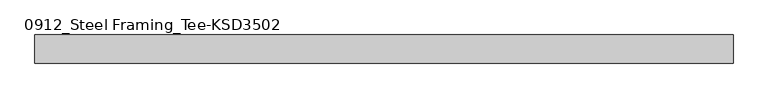
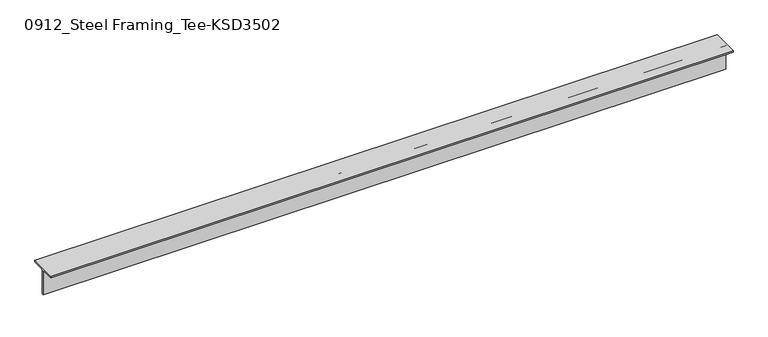
"""IFC4 building model written with IfcOpenShell, lengths in millimetres: member geometry, 0912_Steel Framing_Tee-KSD3502 : H_SB_ASB_CT-150x150x6.5x9."""

from ifc_helpers import new_model, si_unit, point, frame, frame_2d, origin, place, context, project, spatial, polyline, circle_curve, trimmed, segment, composite_curve, outline, extrude, source, transform, mapped, element, save


def member_0912_steel_framing_tee_ksd3502_bae0200a(model_context):
    return source(origin(), model_context, "Body", "SweptSolid", [
        extrude(outline(composite_curve([segment(polyline([(-75.0, 75.0), (75.0, 75.0), (75.0, 66.0), (16.25, 66.0)]), True, "CONTINUOUS"), segment(trimmed(circle_curve(frame_2d((16.25, 53.0)), 13.0), [point((16.25, 66.0))], [point((3.25, 53.0))], True, "CARTESIAN"), True, "CONTINUOUS"), segment(polyline([(3.25, 53.0), (3.25, -75.0), (-3.25, -75.0), (-3.25, 53.0)]), True, "CONTINUOUS"), segment(trimmed(circle_curve(frame_2d((-16.25, 53.0)), 13.0), [point((-3.25, 53.0))], [point((-16.25, 66.0))], True, "CARTESIAN"), True, "CONTINUOUS"), segment(polyline([(-16.25, 66.0), (-75.0, 66.0), (-75.0, 75.0)]), True, "CONTINUOUS")], self_intersect=False)), frame((-1887.85, 0.0, 0.0), z_axis=(1.0, 0.0, 0.0), x_axis=(0.0, 1.0, 0.0)), (0.0, 0.0, 1.0), 3728.1),
    ])


if __name__ == "__main__":
    model = new_model("IFC4")
    model_context = context("Model", 3, world=origin())
    ifc_project = project(units=[si_unit("LENGTHUNIT", "METRE", prefix="MILLI")], contexts=[model_context])
    site = spatial("IfcSite", under=ifc_project)
    building = spatial("IfcBuilding", under=site)
    placement = place(None, origin())
    member_0912_steel_framing_tee_ksd3502_shape = member_0912_steel_framing_tee_ksd3502_bae0200a(model_context)
    element("IfcMember", 1, ObjectType="0912_Steel Framing_Tee-KSD3502 : H_SB_ASB_CT-150x150x6.5x9", at=placement, inside=building, context=model_context, shape_type="MappedRepresentation", body=[
        mapped(member_0912_steel_framing_tee_ksd3502_shape, transform((0.0, 0.0, 0.0), x_axis=(1.0, 0.0, 0.0), y_axis=(0.0, 1.0, 0.0), z_axis=(0.0, 0.0, 1.0))),
    ])
    save(model, "model.ifc")

# Revit data of these elements
# Type "0912_Steel Framing_Tee-KSD3502 : H_SB_ASB_CT-150x150x6.5x9"
#   H_WM Code_1 = "S01AA003-00001 | Main Steel Structure Fabrication Work | Shelter/Building | Light Steel - Standard (30KG/M>Weight) | Material: (   )"
#   H_WM Code_2 = "S03AA029-00001 | Main Steel Structure Erection Work | Shelter/Building | Light Steel (30KG/M>Weight) | Material: (   )"
#   H_WM Code_3 = "S01AA010-00001 | Main Steel Structure Fabrication Work | Shelter/Building | Steel Painting/Coating | for Non-Fireproofed Steel Surface, Surface Preparation, Primer, Second & Final Coat | Material: (   )"
#   H_Q'ty Cal Type Tag = "SB-Q2"
#   Width = 15.0 cm
#   Web Thickness = 0.65 cm
#   Web Fillet = 1.3 cm
#   Section Area = 23.39 cm²
#   Perimeter = 0.60 m²/m
#   Nominal Weight = 18.40 kgf/m
#   Height = 15.0 cm
#   Flange Thickness = 0.9 cm
#   Centroid Vertical = 7.5 cm
#   Centroid Horizontal = 7.5 cm
#   Length [instance default] = 1.5000 m
#   Structural Material [instance default] = Steel, 45-345
#   Warping Constant = (empty or 0)
#   Torsional Moment of Inertia = 0
#   Section Name Key = ""
#   Plastic Modulus weak axis = 0
#   Plastic Modulus strong axis = 0
#   Moment of Inertia weak axis = 0
#   Moment of Inertia strong axis = 0
#   Elastic Modulus weak axis = 0
#   Elastic Modulus strong axis = 0
#   Bolt Spacing = 0
#   Assembly Code = ""
# Element 1 (IfcMember, "0912_Steel Framing_Tee-KSD3502 : H_SB_ASB_CT-150x150x6.5x9")
#   Structural Material = none
# Materials
#   "Steel, 45-345": class "Metal", colour RGB 189 187 185, transparency 0, Description = "Steel 345 MPa", Cost = 0
